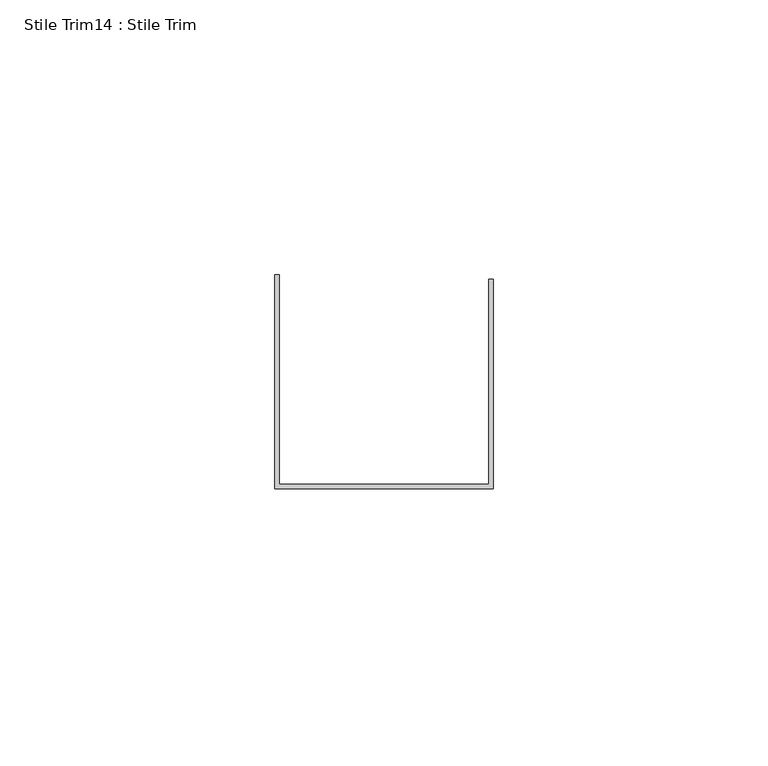
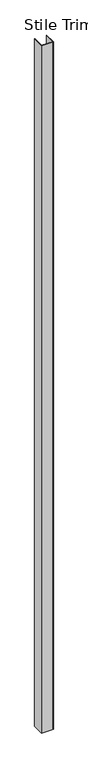
"""IFC4 building model written with IfcOpenShell, lengths in millimetres: proxy geometry, Stile Trim14 : Stile Trim."""

from ifc_helpers import new_model, si_unit, frame, origin, place, context, project, spatial, polyline, outline, extrude, source, transform, mapped, element, save


def stile_trim14_stile_trim_c821ec75(model_context):
    return source(origin(), model_context, "Body", "SweptSolid", [
        extrude(outline(polyline([(587327.0060739, -534097.4537841), (587327.0060739, -534058.5663841), (587327.7934739, -534058.5663841), (587327.7934739, -534096.6663841), (587365.8934739, -534096.6663841), (587365.8934739, -534059.3537841), (587366.6808739, -534059.3537841), (587366.6808739, -534097.4537841), (587327.0060739, -534097.4537841)])), frame((0.0, 0.0, 12.7), z_axis=(0.0, 0.0, 1.0), x_axis=(1.0, 0.0, 0.0)), (0.0, 0.0, 1.0), 2425.7),
    ])


if __name__ == "__main__":
    model = new_model("IFC4")
    model_context = context("Model", 3, world=origin())
    ifc_project = project(units=[si_unit("LENGTHUNIT", "METRE", prefix="MILLI")], contexts=[model_context])
    site = spatial("IfcSite", under=ifc_project)
    building = spatial("IfcBuilding", under=site)
    placement = place(None, origin())
    stile_trim14_stile_trim_shape = stile_trim14_stile_trim_c821ec75(model_context)
    element("IfcBuildingElementProxy", 1, Name="Stile Trim14 : Stile Trim", ObjectType="Stile Trim14 : Stile Trim", at=placement, inside=building, context=model_context, shape_type="MappedRepresentation", body=[
        mapped(stile_trim14_stile_trim_shape, transform((0.0, 0.0, 0.0), x_axis=(1.0, 0.0, 0.0), y_axis=(0.0, 1.0, 0.0), z_axis=(0.0, 0.0, 1.0))),
    ])
    save(model, "model.ifc")

# Revit data of these elements
# Element 1 (IfcBuildingElementProxy, "Stile Trim14 : Stile Trim")
#   Materials on its faces: "EDGE TRIM BY MTL PANEL MFR."
# Materials
#   "EDGE TRIM BY MTL PANEL MFR.": class "Generic", colour RGB 239 242 240, transparency 0, Cost = 0
